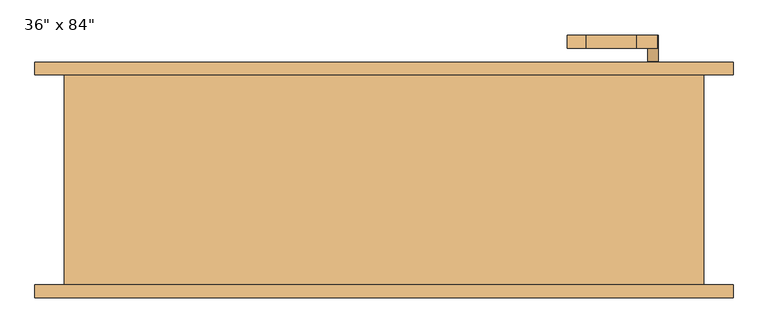
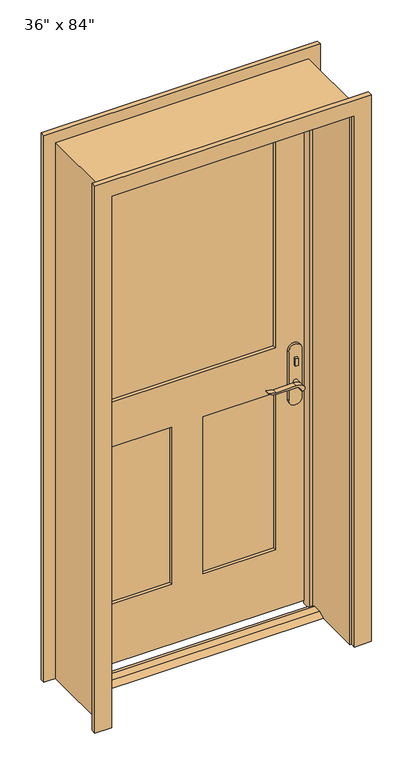
"""IFC4 building model written with IfcOpenShell, lengths in millimetres: door geometry."""

from ifc_helpers import new_model, si_unit, point, frame, frame_2d, origin, place, context, project, spatial, polyline, circle_curve, trimmed, segment, composite_curve, outline, extrude, faceted_brep, source, transform, mapped, element, save


def door_d8dbf45d(model_context):
    return source(origin(), model_context, "Body", "SolidModel", [
        extrude(outline(polyline([(38.1, 12.7), (73.025, 12.7), (98.425, 0.0), (12.7, 0.0), (38.1, 12.7)])), frame((-457.2, 0.0, 0.0), z_axis=(1.0, 0.0, 0.0), x_axis=(0.0, 1.0, 0.0)), (0.0, 0.0, 1.0), 914.4),
        extrude(outline(polyline([(411.4, 100.65), (401.4, 100.65), (401.4, 110.65), (411.4, 110.65), (411.4, 100.65)])), frame((0.0, 0.0, 981.9), z_axis=(0.0, 0.0, 1.0), x_axis=(1.0, 0.0, 0.0)), (0.0, 0.0, 1.0), 30.0),
        extrude(outline(composite_curve([segment(trimmed(circle_curve(frame_2d((996.9, 406.4)), 8.0), [point((996.9, 398.4))], [point((996.9, 414.4))], False, "CARTESIAN"), True, "CONTINUOUS"), segment(trimmed(circle_curve(frame_2d((996.9, 406.4)), 8.0), [point((996.9, 414.4))], [point((996.9, 398.4))], False, "CARTESIAN"), True, "CONTINUOUS")], self_intersect=False)), frame((0.0, 165.575, 0.0), z_axis=(0.0, 1.0, 0.0), x_axis=(0.0, 0.0, 1.0)), (0.0, 0.0, 1.0), 10.0),
        extrude(outline(composite_curve([segment(trimmed(circle_curve(frame_2d((897.1555521, 382.7324871)), 37.2832219), [point((919.0523287, 412.9081363))], [point((934.4, 381.0325667))], False, "CARTESIAN"), True, "CONTINUOUS"), segment(polyline([(934.4, 381.0325667), (934.4, 304.7564091)]), True, "CONTINUOUS"), segment(trimmed(circle_curve(frame_2d((1017.6850638, 304.8227909)), 83.2850902), [point((934.4, 304.7564091))], [point((939.4, 276.4))], True, "CARTESIAN"), True, "CONTINUOUS"), segment(polyline([(939.4, 276.4), (936.6135558, 276.4)]), True, "CONTINUOUS"), segment(trimmed(circle_curve(frame_2d((986.6709207, 308.3396612)), 59.3791355), [point((936.6135558, 276.4))], [point((927.4, 304.7564091))], False, "CARTESIAN"), True, "CONTINUOUS"), segment(polyline([(927.4, 304.7564091), (927.4, 381.0138099)]), True, "CONTINUOUS"), segment(trimmed(circle_curve(frame_2d((909.2738613, 381.0138099)), 18.1261387), [point((927.4, 381.0138099))], [point((914.4, 398.4))], True, "CARTESIAN"), True, "CONTINUOUS"), segment(trimmed(circle_curve(frame_2d((914.4, 406.4)), 8.0), [point((914.4, 398.4))], [point((919.0523287, 412.9081363))], False, "CARTESIAN"), True, "CONTINUOUS")], self_intersect=False)), frame((0.0, 60.65, 0.0), z_axis=(0.0, 1.0, 0.0), x_axis=(0.0, 0.0, 1.0)), (0.0, 0.0, 1.0), 20.0),
        extrude(outline(composite_curve([segment(trimmed(circle_curve(frame_2d((914.4, 406.4)), 8.0), [point((914.3999903, 398.4))], [point((919.0523287, 412.9081363))], False, "CARTESIAN"), True, "CONTINUOUS"), segment(trimmed(circle_curve(frame_2d((897.1555521, 382.7324871)), 37.2832219), [point((919.0523287, 412.9081363))], [point((934.4, 381.0325667))], False, "CARTESIAN"), True, "CONTINUOUS"), segment(polyline([(934.4, 381.0325667), (934.4, 304.7564091)]), True, "CONTINUOUS"), segment(trimmed(circle_curve(frame_2d((1017.6850638, 304.8227909)), 83.2850902), [point((934.4, 304.7564091))], [point((939.4, 276.4))], True, "CARTESIAN"), True, "CONTINUOUS"), segment(polyline([(939.4, 276.4), (936.6135558, 276.4)]), True, "CONTINUOUS"), segment(trimmed(circle_curve(frame_2d((986.6709207, 308.3396612)), 59.3791355), [point((936.6135558, 276.4))], [point((927.4, 304.7564091))], False, "CARTESIAN"), True, "CONTINUOUS"), segment(polyline([(927.4, 304.7564091), (927.4, 381.0138122)]), True, "CONTINUOUS"), segment(trimmed(circle_curve(frame_2d((909.2738682, 381.0138122)), 18.1261318), [point((927.4, 381.0138122))], [point((914.3999903, 398.4))], True, "CARTESIAN"), True, "CONTINUOUS")], self_intersect=False)), frame((0.0, 195.575, 0.0), z_axis=(0.0, 1.0, 0.0), x_axis=(0.0, 0.0, 1.0)), (0.0, 0.0, 1.0), 20.0),
        extrude(outline(composite_curve([segment(trimmed(circle_curve(frame_2d((914.4, 406.4)), 8.0), [point((914.4, 398.4))], [point((914.4, 414.4))], False, "CARTESIAN"), True, "CONTINUOUS"), segment(trimmed(circle_curve(frame_2d((914.4, 406.4)), 8.0), [point((914.4, 414.4))], [point((914.4, 398.4))], False, "CARTESIAN"), True, "CONTINUOUS")], self_intersect=False)), frame((0.0, 80.65, 0.0), z_axis=(0.0, 1.0, 0.0), x_axis=(0.0, 0.0, 1.0)), (0.0, 0.0, 1.0), 30.0),
        extrude(outline(composite_curve([segment(trimmed(circle_curve(frame_2d((914.4, 406.4)), 8.0), [point((914.4, 398.4))], [point((914.4, 414.4))], False, "CARTESIAN"), True, "CONTINUOUS"), segment(trimmed(circle_curve(frame_2d((914.4, 406.4)), 8.0), [point((914.4, 414.4))], [point((914.4, 398.4))], False, "CARTESIAN"), True, "CONTINUOUS")], self_intersect=False)), frame((0.0, 165.575, 0.0), z_axis=(0.0, 1.0, 0.0), x_axis=(0.0, 0.0, 1.0)), (0.0, 0.0, 1.0), 30.0),
        extrude(outline(composite_curve([segment(polyline([(844.4, 431.4), (1039.4, 431.4)]), True, "CONTINUOUS"), segment(trimmed(circle_curve(frame_2d((1039.4, 406.4)), 25.0), [point((1039.4, 431.4))], [point((1039.4, 381.4))], False, "CARTESIAN"), True, "CONTINUOUS"), segment(polyline([(1039.4, 381.4), (844.4, 381.4)]), True, "CONTINUOUS"), segment(trimmed(circle_curve(frame_2d((844.4, 406.4)), 25.0), [point((844.4, 381.4))], [point((844.4, 431.4))], False, "CARTESIAN"), True, "CONTINUOUS")], self_intersect=False)), frame((0.0, 110.65, 0.0), z_axis=(0.0, 1.0, 0.0), x_axis=(0.0, 0.0, 1.0)), (0.0, 0.0, 1.0), 10.0),
        extrude(outline(composite_curve([segment(polyline([(844.4, 431.4), (1039.4, 431.4)]), True, "CONTINUOUS"), segment(trimmed(circle_curve(frame_2d((1039.4, 406.4)), 25.0), [point((1039.4, 431.4))], [point((1039.4, 381.4))], False, "CARTESIAN"), True, "CONTINUOUS"), segment(polyline([(1039.4, 381.4), (844.4, 381.4)]), True, "CONTINUOUS"), segment(trimmed(circle_curve(frame_2d((844.4, 406.4)), 25.0), [point((844.4, 381.4))], [point((844.4, 431.4))], False, "CARTESIAN"), True, "CONTINUOUS")], self_intersect=False)), frame((0.0, 155.575, 0.0), z_axis=(0.0, 1.0, 0.0), x_axis=(0.0, 0.0, 1.0)), (0.0, 0.0, 1.0), 10.0),
        extrude(outline(polyline([(2133.6, -457.2), (12.7, -457.2), (12.7, 457.2), (2133.6, 457.2), (2133.6, -457.2)]), holes=[polyline([(1066.8, -336.55), (2012.95, -336.55), (2012.95, 336.55), (1066.8, 336.55), (1066.8, -336.55)]), polyline([(885.825, -60.325), (254.0, -60.325), (254.0, -336.55), (885.825, -336.55), (885.825, -60.325)]), polyline([(885.825, 336.55), (254.0, 336.55), (254.0, 60.325), (885.825, 60.325), (885.825, 336.55)])]), frame((0.0, 120.65, 0.0), z_axis=(0.0, 1.0, 0.0), x_axis=(0.0, 0.0, 1.0)), (0.0, 0.0, 1.0), 34.925),
        faceted_brep([(482.6, 155.575, 0.0), (482.6, -161.925, 0.0), (457.2, -161.925, 0.0), (457.2, 85.725, 0.0), (444.5, 85.725, 0.0), (444.5, 120.65, 0.0), (457.2, 120.65, 0.0), (457.2, 155.575, 0.0), (482.6, 155.575, 2159.0), (482.6, -161.925, 2159.0), (-482.6, -161.925, 2159.0), (-482.6, -161.925, 0.0), (-457.2, -161.925, 0.0), (-457.2, -161.925, 2133.6), (457.2, -161.925, 2133.6), (457.2, 85.725, 2133.6), (-457.2, 85.725, 2133.6), (-457.2, 85.725, 0.0), (-444.5, 85.725, 0.0), (-444.5, 85.725, 2120.9), (444.5, 85.725, 2120.9), (444.5, 120.65, 2120.9), (-444.5, 120.65, 2120.9), (-444.5, 120.65, 0.0), (-457.2, 120.65, 0.0), (-457.2, 120.65, 2133.6), (457.2, 120.65, 2133.6), (457.2, 155.575, 2133.6), (-457.2, 155.575, 2133.6), (-457.2, 155.575, 0.0), (-482.6, 155.575, 0.0), (-482.6, 155.575, 2159.0)], [[[0, 1, 2, 3, 4, 5, 6, 7]], [[1, 0, 8, 9]], [[2, 1, 9, 10, 11, 12, 13, 14]], [[3, 2, 14, 15]], [[4, 3, 15, 16, 17, 18, 19, 20]], [[5, 4, 20, 21]], [[6, 5, 21, 22, 23, 24, 25, 26]], [[7, 6, 26, 27]], [[0, 7, 27, 28, 29, 30, 31, 8]], [[9, 8, 31, 10]], [[15, 14, 13, 16]], [[21, 20, 19, 22]], [[27, 26, 25, 28]], [[30, 29, 24, 23, 18, 17, 12, 11]], [[10, 31, 30, 11]], [[16, 13, 12, 17]], [[22, 19, 18, 23]], [[28, 25, 24, 29]]]),
        extrude(outline(polyline([(-60.325, 132.2916667), (-336.55, 132.2916667), (-336.55, 143.9333333), (-60.325, 143.9333333), (-60.325, 132.2916667)])), frame((0.0, 0.0, 254.0), z_axis=(0.0, 0.0, 1.0), x_axis=(1.0, 0.0, 0.0)), (0.0, 0.0, 1.0), 631.825),
        extrude(outline(polyline([(336.55, 132.2916667), (60.325, 132.2916667), (60.325, 143.9333333), (336.55, 143.9333333), (336.55, 132.2916667)])), frame((0.0, 0.0, 254.0), z_axis=(0.0, 0.0, 1.0), x_axis=(1.0, 0.0, 0.0)), (0.0, 0.0, 1.0), 631.825),
        extrude(outline(polyline([(336.55, 134.62), (-336.55, 134.62), (-336.55, 141.605), (336.55, 141.605), (336.55, 134.62)])), frame((0.0, 0.0, 1066.8), z_axis=(0.0, 0.0, 1.0), x_axis=(1.0, 0.0, 0.0)), (0.0, 0.0, 1.0), 946.15),
        extrude(outline(polyline([(0.0, -527.05), (0.0, -463.55), (2139.95, -463.55), (2139.95, 463.55), (0.0, 463.55), (0.0, 527.05), (2203.45, 527.05), (2203.45, -527.05), (0.0, -527.05)])), frame((0.0, -180.975, 0.0), z_axis=(0.0, 1.0, 0.0), x_axis=(0.0, 0.0, 1.0)), (0.0, 0.0, 1.0), 19.05),
        extrude(outline(polyline([(0.0, -527.05), (0.0, -463.55), (2139.95, -463.55), (2139.95, 463.55), (0.0, 463.55), (0.0, 527.05), (2203.45, 527.05), (2203.45, -527.05), (0.0, -527.05)])), frame((0.0, 155.575, 0.0), z_axis=(0.0, 1.0, 0.0), x_axis=(0.0, 0.0, 1.0)), (0.0, 0.0, 1.0), 19.05),
    ])


if __name__ == "__main__":
    model = new_model("IFC4")
    model_context = context("Model", 3, world=origin())
    ifc_project = project(units=[si_unit("LENGTHUNIT", "METRE", prefix="MILLI")], contexts=[model_context])
    site = spatial("IfcSite", under=ifc_project)
    building = spatial("IfcBuilding", under=site)
    placement = place(None, origin())
    door_shape = door_d8dbf45d(model_context)
    element("IfcDoor", 1, ObjectType="Door-Exterior-Single-Entry-Half Flat Glass-Wood_Clad : 36\" x 84\"", at=placement, inside=building, context=model_context, shape_type="MappedRepresentation", body=[
        mapped(door_shape, transform((0.0, 0.0, 0.0), x_axis=(1.0, 0.0, 0.0), y_axis=(0.0, 1.0, 0.0), z_axis=(0.0, 0.0, 1.0))),
    ])
    save(model, "model.ifc")

# Revit data of these elements
# Type "Door-Exterior-Single-Entry-Half Flat Glass-Wood_Clad : 36\" x 84\""
#   Type Mark = "25"
#   Assembly Code = "B2030100"
#   Analytic Construction = "French door, wood frame with single glass"
#   Top Rail = 0' - 4 3/4"
#   Threshold Offset [instance default] = 0' - 0 1/2"
#   Thickness = 0' - 1 3/8"
#   Thermal Resistance (R) = 1.0696 (h·ft²·°F)/BTU
#   Swing Angle [instance default] = 90.0000°
#   Stiles = 0' - 4 3/4"
#   Rough Width = 3' - 2"
#   Rough Height = 7' - 1"
#   Lock Rail = 0' - 7 1/8"
#   Height = 7' - 0"
#   Width = 3' - 0"
#   Heat Transfer Coefficient (U) = 0.9350 BTU/(h·ft²·°F)
#   Door Offset [instance default] = 0' - 0"
#   Bottom Rail = 0' - 9 1/2"
#   Threshold [instance default] = yes
#   Function = 1
#   Exterior Trim [instance default] = yes
#   Trim Material = Glass, Clear Glazing
#   Threshold Material = Maple - Semigloss(Rotated)
#   Panel Material = Clad - White
#   Glazing = Glass, Clear Glazing
#   Frame Material = Clad - White
#   Door Handle Material = Aluminum
#   Visual Light Transmittance = 0
#   Solar Heat Gain Coefficient = 0
#   Wall Closure = (empty or 0)
#   Construction Type = (empty or 0)
# Element 1 (IfcDoor, "Door-Exterior-Single-Entry-Half Flat Glass-Wood_Clad : 36\" x 84\"")
#   Materials on its faces: "Aluminum", "Clad - White", "Glass, Clear Glazing", "Maple - Semigloss(Rotated)"
# Materials
#   "Glass, Clear Glazing": class "Glass", colour RGB 245 245 243, transparency 1, Description = "Clear glazing", Cost = 0
#   "Maple - Semigloss(Rotated)": class "Wood", colour RGB 196 161 118, transparency 0, Description = "Acer Saccharum", Cost = 0
#   "Clad - White": class "Wood", colour RGB 245 245 243, transparency 0, Cost = 0
#   "Aluminum": class "Metal", colour RGB 244 245 246, transparency 0, Description = "Aluminum 6061", Cost = 0
